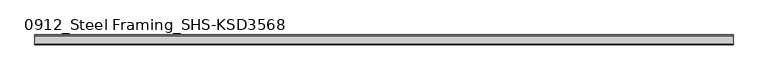
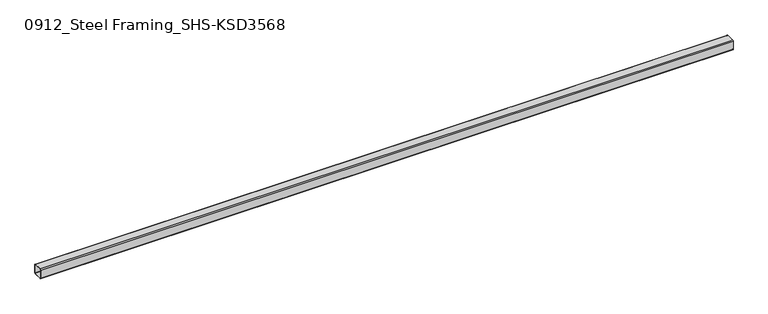
"""IFC4 building model written with IfcOpenShell, lengths in millimetres: beam geometry, 0912_Steel Framing_SHS-KSD3568 : H_SB_ASB_SHS-150x150x6."""

from ifc_helpers import new_model, si_unit, point, frame, frame_2d, origin, place, context, project, spatial, polyline, circle_curve, trimmed, segment, composite_curve, outline, extrude, source, transform, mapped, element, save


def beam_0912_steel_framing_shs_ksd3568_00c61770(model_context):
    return source(origin(), model_context, "Body", "SweptSolid", [
        extrude(outline(composite_curve([segment(trimmed(circle_curve(frame_2d((-63.0, 63.0)), 12.0), [point((-75.0, 63.0))], [point((-63.0, 75.0))], False, "CARTESIAN"), True, "CONTINUOUS"), segment(polyline([(-63.0, 75.0), (63.0, 75.0)]), True, "CONTINUOUS"), segment(trimmed(circle_curve(frame_2d((63.0, 63.0)), 12.0), [point((63.0, 75.0))], [point((75.0, 63.0))], False, "CARTESIAN"), True, "CONTINUOUS"), segment(polyline([(75.0, 63.0), (75.0, -63.0)]), True, "CONTINUOUS"), segment(trimmed(circle_curve(frame_2d((63.0, -63.0)), 12.0), [point((75.0, -63.0))], [point((63.0, -75.0))], False, "CARTESIAN"), True, "CONTINUOUS"), segment(polyline([(63.0, -75.0), (-63.0, -75.0)]), True, "CONTINUOUS"), segment(trimmed(circle_curve(frame_2d((-63.0, -63.0)), 12.0), [point((-63.0, -75.0))], [point((-75.0, -63.0))], False, "CARTESIAN"), True, "CONTINUOUS"), segment(polyline([(-75.0, -63.0), (-75.0, 63.0)]), True, "CONTINUOUS")], self_intersect=False), holes=[composite_curve([segment(polyline([(63.0, 69.0), (-63.0, 69.0)]), True, "CONTINUOUS"), segment(trimmed(circle_curve(frame_2d((-63.0, 63.0)), 6.0), [point((-63.0, 69.0))], [point((-69.0, 63.0))], True, "CARTESIAN"), True, "CONTINUOUS"), segment(polyline([(-69.0, 63.0), (-69.0, -63.0)]), True, "CONTINUOUS"), segment(trimmed(circle_curve(frame_2d((-63.0, -63.0)), 6.0), [point((-69.0, -63.0))], [point((-63.0, -69.0))], True, "CARTESIAN"), True, "CONTINUOUS"), segment(polyline([(-63.0, -69.0), (63.0, -69.0)]), True, "CONTINUOUS"), segment(trimmed(circle_curve(frame_2d((63.0, -63.0)), 6.0), [point((63.0, -69.0))], [point((69.0, -63.0))], True, "CARTESIAN"), True, "CONTINUOUS"), segment(polyline([(69.0, -63.0), (69.0, 63.0)]), True, "CONTINUOUS"), segment(trimmed(circle_curve(frame_2d((63.0, 63.0)), 6.0), [point((69.0, 63.0))], [point((63.0, 69.0))], True, "CARTESIAN"), True, "CONTINUOUS")], self_intersect=False)]), frame((-5215.0, 0.0, 0.0), z_axis=(1.0, 0.0, 0.0), x_axis=(0.0, 1.0, 0.0)), (0.0, 0.0, 1.0), 10430.0),
    ])


if __name__ == "__main__":
    model = new_model("IFC4")
    model_context = context("Model", 3, world=origin())
    ifc_project = project(units=[si_unit("LENGTHUNIT", "METRE", prefix="MILLI")], contexts=[model_context])
    site = spatial("IfcSite", under=ifc_project)
    building = spatial("IfcBuilding", under=site)
    placement = place(None, origin())
    beam_0912_steel_framing_shs_ksd3568_shape = beam_0912_steel_framing_shs_ksd3568_00c61770(model_context)
    element("IfcBeam", 1, ObjectType="0912_Steel Framing_SHS-KSD3568 : H_SB_ASB_SHS-150x150x6", at=placement, inside=building, context=model_context, shape_type="MappedRepresentation", body=[
        mapped(beam_0912_steel_framing_shs_ksd3568_shape, transform((0.0, 0.0, 0.0), x_axis=(1.0, 0.0, 0.0), y_axis=(0.0, 1.0, 0.0), z_axis=(0.0, 0.0, 1.0))),
    ])
    save(model, "model.ifc")

# Revit data of these elements
# Type "0912_Steel Framing_SHS-KSD3568 : H_SB_ASB_SHS-150x150x6"
#   H_WM Code_1 = "S01AA002-00001 | Main Steel Structure Fabrication Work | Shelter/Building | Medium Steel - Standard (90KG/M>Weight≥30KG/M) | Material: (   )"
#   H_WM Code_2 = "S03AA028-00001 | Main Steel Structure Erection Work | Shelter/Building | Medium Steel (90KG/M>Weight≥30KG/M) | Material: (   )"
#   H_WM Code_3 = "S01AA010-00001 | Main Steel Structure Fabrication Work | Shelter/Building | Steel Painting/Coating | for Non-Fireproofed Steel Surface, Surface Preparation, Primer, Second & Final Coat | Material: (   )"
#   H_Q'ty Cal Type Tag = "SB-Q2"
#   Perimeter = 0.60 m²/m
#   Nominal Weight = 26.40 kgf/m
#   Length [instance default] = 1.0000 m
#   b = 0.1500 m
#   h = 0.1500 m
#   tr = 0.0120 m
#   t = 0.0060 m
#   A = 28.36 m²
#   Structural Material [instance default] = Steel, 45-345
# Element 1 (IfcBeam, "0912_Steel Framing_SHS-KSD3568 : H_SB_ASB_SHS-150x150x6")
#   Structural Material = none
# Materials
#   "Steel, 45-345": class "Metal", colour RGB 189 187 185, transparency 0, Description = "Steel 345 MPa", Cost = 0
